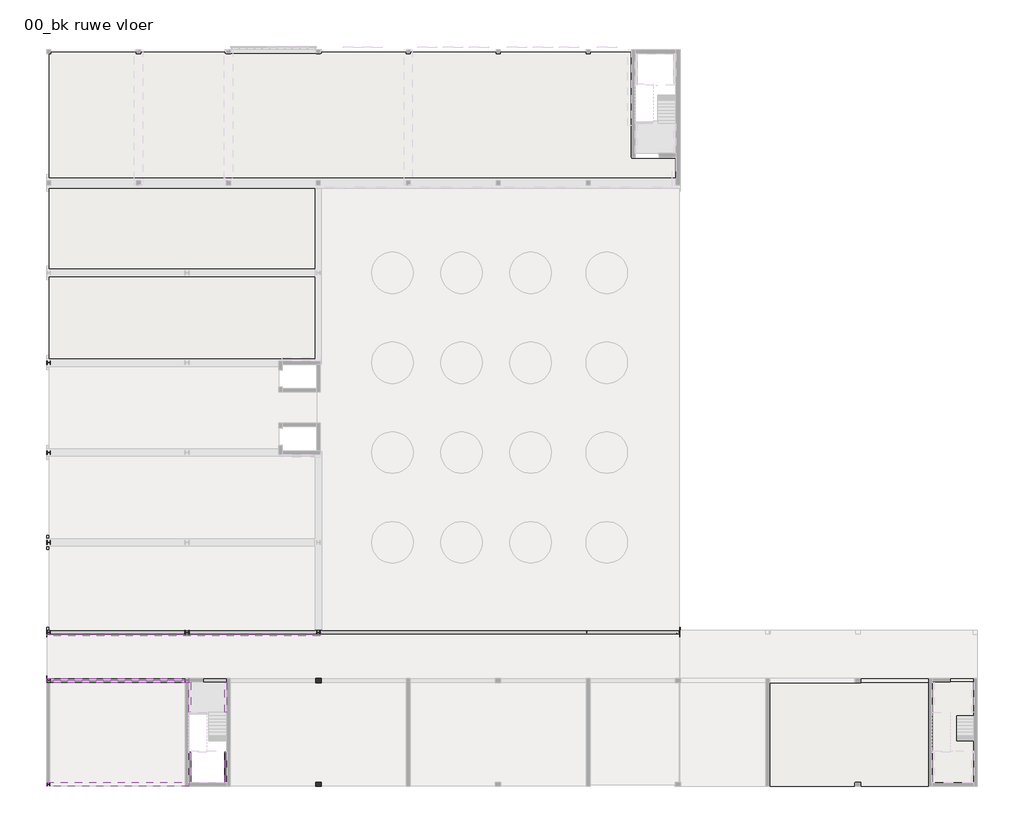
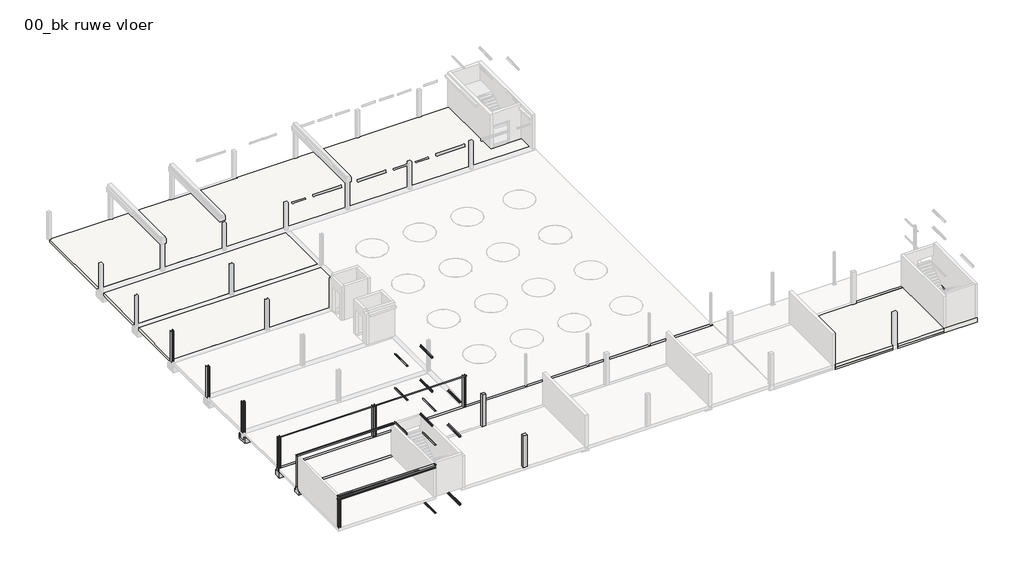
# One storey, part 4 of 6: 24 beams, 10 columns, 8 slabs.
"""IFC4 building model written with IfcOpenShell, lengths in millimetres."""

import ifcopenshell
import ifcopenshell.guid

model = None  # the IFC model being written
_history = None  # IfcOwnerHistory: only IFC2X3 demands one
_inside = {}  # id of a spatial element -> (the spatial element, [elements in it])
_under = {}  # id of a project, library or spatial element -> (it, [spatial elements below it])
_declared = {}  # id of a project -> (the project, [libraries it declares])
_typed = {}  # id of a type object -> (the type object, [elements of that type])
_made_of = {}  # id of a material, layer set ... -> (it, [elements and type objects made of it])


def new_model(schema):
    """Start an empty IFC model of exactly this schema.

    Asked for "IFC4X3", IfcOpenShell would pick the latest addendum, in which some entities
    have other attributes; the version numbers below select the first issue.
    IFC2X3 requires an IfcOwnerHistory on every rooted entity: one is made here for all.
    """
    global model, _history
    if schema == "IFC4X3":
        model = ifcopenshell.file(schema_version=(4, 3, 0, 0))
    else:
        model = ifcopenshell.file(schema=schema)
    _inside.clear()
    _under.clear()
    _declared.clear()
    _typed.clear()
    _made_of.clear()
    _history = None
    if model.schema == "IFC2X3":
        org = make("IfcOrganization", Name="unknown")
        user = make(
            "IfcPersonAndOrganization",
            ThePerson=make("IfcPerson", FamilyName="unknown"),
            TheOrganization=org,
        )
        app = make(
            "IfcApplication",
            ApplicationDeveloper=org,
            Version="unknown",
            ApplicationFullName="unknown",
            ApplicationIdentifier="unknown",
        )
        _history = make(
            "IfcOwnerHistory",
            OwningUser=user,
            OwningApplication=app,
            ChangeAction="ADDED",
            CreationDate=0,
        )
    return model


def make(cls, **values):
    """One entity of the class cls with the attributes given. An attribute that is None is left unset."""
    return model.create_entity(
        cls, **{name: value for name, value in values.items() if value is not None}
    )


def rooted(cls, **values):
    """An entity with a GlobalId (a new one), such as an element, a storey or a relation."""
    return make(cls, GlobalId=ifcopenshell.guid.new(), OwnerHistory=_history, **values)


def si_unit(unit_type, name, prefix=None):
    """IfcSIUnit, for example si_unit("LENGTHUNIT", "METRE", prefix="MILLI")."""
    return make("IfcSIUnit", UnitType=unit_type, Prefix=prefix, Name=name)


def assignment(units):
    """IfcUnitAssignment: the units of a project."""
    return None if units is None else make("IfcUnitAssignment", Units=units)


def point(xyz):
    """IfcCartesianPoint."""
    return None if xyz is None else make("IfcCartesianPoint", Coordinates=xyz)


def direction(xyz):
    """IfcDirection."""
    return None if xyz is None else make("IfcDirection", DirectionRatios=xyz)


def frame(location, z_axis=None, x_axis=None):
    """IfcAxis2Placement3D, a coordinate frame: its origin and axes. An axis left out is left unset."""
    return make(
        "IfcAxis2Placement3D",
        Location=point(location),
        Axis=direction(z_axis),
        RefDirection=direction(x_axis),
    )


def frame_2d(location, x_axis=None):
    """IfcAxis2Placement2D, a coordinate frame in the plane: its origin and x axis."""
    return make(
        "IfcAxis2Placement2D", Location=point(location), RefDirection=direction(x_axis)
    )


def origin():
    """The frame at (0, 0, 0) with its axes left unset."""
    return frame((0.0, 0.0, 0.0))


def place(relative_to, where):
    """IfcLocalPlacement: puts the frame where relative to a parent placement (None: the world)."""
    return make(
        "IfcLocalPlacement", PlacementRelTo=relative_to, RelativePlacement=where
    )


def context(
    kind, dimensions, precision=None, world=None, true_north=None, identifier=None
):
    """IfcGeometricRepresentationContext, for example the 3D "Model" context."""
    return make(
        "IfcGeometricRepresentationContext",
        ContextIdentifier=identifier,
        ContextType=kind,
        CoordinateSpaceDimension=dimensions,
        Precision=precision,
        WorldCoordinateSystem=world,
        TrueNorth=true_north,
    )


def project(units=None, contexts=None):
    """IfcProject with its units and contexts."""
    return rooted(
        "IfcProject",
        Name="project",
        RepresentationContexts=contexts,
        UnitsInContext=assignment(units),
    )


def spatial(cls, under=None, at=None, **own):
    """A site, building, storey or space (cls), placed at a placement, below another one or the project."""
    s = rooted(cls, ObjectPlacement=at, **own)
    if under is not None:
        _under.setdefault(under.id(), (under, []))[1].append(s)
    return s


def polyline(points):
    """IfcPolyline through the points."""
    return make("IfcPolyline", Points=[point(p) for p in points])


def circle_curve(where, radius):
    """IfcCircle in the frame where."""
    return make("IfcCircle", Position=where, Radius=radius)


def trimmed(basis, trim1, trim2, sense, master):
    """IfcTrimmedCurve: the piece of a basis curve between two trims."""
    return make(
        "IfcTrimmedCurve",
        BasisCurve=basis,
        Trim1=trim1,
        Trim2=trim2,
        SenseAgreement=sense,
        MasterRepresentation=master,
    )


def segment(curve, same_sense, transition):
    """IfcCompositeCurveSegment."""
    return make(
        "IfcCompositeCurveSegment",
        Transition=transition,
        SameSense=same_sense,
        ParentCurve=curve,
    )


def composite_curve(segments, self_intersect=None):
    """IfcCompositeCurve: segments joined end to end."""
    return make("IfcCompositeCurve", Segments=segments, SelfIntersect=self_intersect)


def outline(outer, holes=None, kind="AREA"):
    """IfcArbitraryClosedProfileDef: a profile drawn as a closed curve; with holes, ...WithVoids."""
    if holes is None:
        return make("IfcArbitraryClosedProfileDef", ProfileType=kind, OuterCurve=outer)
    return make(
        "IfcArbitraryProfileDefWithVoids",
        ProfileType=kind,
        OuterCurve=outer,
        InnerCurves=holes,
    )


def extrude(swept, where, along, depth):
    """IfcExtrudedAreaSolid: the profile swept, set in the frame where, extruded along a direction by depth."""
    return make(
        "IfcExtrudedAreaSolid",
        SweptArea=swept,
        Position=where,
        ExtrudedDirection=direction(along),
        Depth=depth,
    )


def faces_of(points, faces, orient=None, outer=None):
    """IfcFace entities. A face is a list of loops; a loop is a list of indices into points, from 0.

    orient and outer hold one flag for each loop. By default every Orientation is true, the
    first loop of a face is its IfcFaceOuterBound and the others are IfcFaceBound.
    """
    made = []
    for i, loops in enumerate(faces):
        bounds = []
        for j, loop in enumerate(loops):
            is_outer = j == 0 if outer is None else outer[i][j]
            bounds.append(
                make(
                    "IfcFaceOuterBound" if is_outer else "IfcFaceBound",
                    Bound=make("IfcPolyLoop", Polygon=[points[k] for k in loop]),
                    Orientation=True if orient is None else orient[i][j],
                )
            )
        made.append(make("IfcFace", Bounds=bounds))
    return made


def faceted_brep(points, faces, orient=None, outer=None, voids=None):
    """IfcFacetedBrep: a solid bounded by flat faces; with voids (closed shells), ...WithVoids."""
    shared = [point(p) for p in points]
    hull = make("IfcClosedShell", CfsFaces=faces_of(shared, faces, orient, outer))
    if voids is None:
        return make("IfcFacetedBrep", Outer=hull)
    return make(
        "IfcFacetedBrepWithVoids",
        Outer=hull,
        Voids=[
            make(cls, CfsFaces=faces_of(shared, fs, o, b)) for cls, fs, o, b in voids
        ],
    )


def shape(context_of_items, identifier, shape_type, items):
    """IfcShapeRepresentation: the items that make up one representation, for example the "Body"."""
    return make(
        "IfcShapeRepresentation",
        ContextOfItems=context_of_items,
        RepresentationIdentifier=identifier,
        RepresentationType=shape_type,
        Items=items,
    )


def source(mapping_origin, context_of_items, identifier, shape_type, items):
    """IfcRepresentationMap: a shape defined once, which mapped items show again and again."""
    return make(
        "IfcRepresentationMap",
        MappingOrigin=mapping_origin,
        MappedRepresentation=shape(context_of_items, identifier, shape_type, items),
    )


def transform(
    local_origin,
    x_axis=None,
    y_axis=None,
    z_axis=None,
    scale=None,
    scale2=None,
    scale3=None,
    uniform=True,
):
    """IfcCartesianTransformationOperator3D, or its non-uniform kind. x_axis, y_axis, z_axis: its Axis1, 2, 3."""
    if uniform:
        return make(
            "IfcCartesianTransformationOperator3D",
            Axis1=direction(x_axis),
            Axis2=direction(y_axis),
            LocalOrigin=point(local_origin),
            Scale=scale,
            Axis3=direction(z_axis),
        )
    return make(
        "IfcCartesianTransformationOperator3DnonUniform",
        Axis1=direction(x_axis),
        Axis2=direction(y_axis),
        LocalOrigin=point(local_origin),
        Scale=scale,
        Axis3=direction(z_axis),
        Scale2=scale2,
        Scale3=scale3,
    )


def mapped(mapping_source, mapping_target):
    """IfcMappedItem: shows the shape of a source again, moved by a transform."""
    return make(
        "IfcMappedItem", MappingSource=mapping_source, MappingTarget=mapping_target
    )


def made_of(thing, what):
    """Note that an element or type object is made of a material, layer set ...; save() writes the relation."""
    if what is not None:
        _made_of.setdefault(what.id(), (what, []))[1].append(thing)
    return thing


def element(
    cls,
    number,
    at=None,
    inside=None,
    cuts=None,
    type_object=None,
    material=None,
    context=None,
    identifier="Body",
    shape_type=None,
    held_by="IfcProductDefinitionShape",
    body=None,
    shapes=None,
    **own,
):
    """One element of the class cls, such as IfcWall. Its Tag is "e" and its number.

    at: its placement. inside: the storey or other place that contains it. cuts: it is an
    opening in that element (IfcRelVoidsElement). A single representation is given by context,
    identifier, shape_type and body (its items); several are given by shapes. held_by: the class
    of the entity that holds the representations. save() writes the other relations.
    """
    e = rooted(cls, Tag="e%d" % number, ObjectPlacement=at, **own)
    if body is not None:
        shapes = [shape(context, identifier, shape_type, body)]
    if shapes is not None:
        e.Representation = make(held_by, Representations=shapes)
    if inside is not None:
        _inside.setdefault(inside.id(), (inside, []))[1].append(e)
    if cuts is not None:
        rooted(
            "IfcRelVoidsElement", RelatingBuildingElement=cuts, RelatedOpeningElement=e
        )
    if type_object is not None:
        _typed.setdefault(type_object.id(), (type_object, []))[1].append(e)
    return made_of(e, material)


def aggregate(whole, parts):
    """IfcRelAggregates: a whole, such as a stair, and the parts it consists of."""
    return rooted("IfcRelAggregates", RelatingObject=whole, RelatedObjects=parts)


def save(model, path):
    """Write the relations noted so far, then the file.

    IfcRelAggregates (storeys below a building ...), IfcRelContainedInSpatialStructure (elements
    in a storey), IfcRelDefinesByType, IfcRelAssociatesMaterial and IfcRelDeclares: one each for
    every whole, place, type object, material and project.
    """
    for whole, parts in _under.values():
        aggregate(whole, parts)
    for where, things in _inside.values():
        rooted(
            "IfcRelContainedInSpatialStructure",
            RelatedElements=things,
            RelatingStructure=where,
        )
    for kind, things in _typed.values():
        rooted("IfcRelDefinesByType", RelatedObjects=things, RelatingType=kind)
    for what, things in _made_of.values():
        rooted("IfcRelAssociatesMaterial", RelatedObjects=things, RelatingMaterial=what)
    for by, libraries in _declared.values():
        rooted("IfcRelDeclares", RelatingContext=by, RelatedDefinitions=libraries)
    model.write(path)


def beam_86464b0d(model_context):
    return source(origin(), model_context, "Body", "SweptSolid", [
        extrude(outline(composite_curve([segment(polyline([(-42.5, -42.5), (-42.5, 107.5), (-35.5, 107.5)]), True, "CONTINUOUS"), segment(trimmed(circle_curve(frame_2d((-35.5, 99.5)), 8.0), [point((-35.5, 107.5))], [point((-27.5, 99.5))], False, "CARTESIAN"), True, "CONTINUOUS"), segment(polyline([(-27.5, 99.5), (-27.5, -11.5)]), True, "CONTINUOUS"), segment(trimmed(circle_curve(frame_2d((-11.5, -11.5)), 16.0), [point((-27.5, -11.5))], [point((-11.5, -27.5))], True, "CARTESIAN"), True, "CONTINUOUS"), segment(polyline([(-11.5, -27.5), (99.5, -27.5)]), True, "CONTINUOUS"), segment(trimmed(circle_curve(frame_2d((99.5, -35.5)), 8.0), [point((99.5, -27.5))], [point((107.5, -35.5))], False, "CARTESIAN"), True, "CONTINUOUS"), segment(polyline([(107.5, -35.5), (107.5, -42.5), (-42.5, -42.5)]), True, "CONTINUOUS")], self_intersect=False)), frame((-1095.0, 0.0, 0.0), z_axis=(1.0, 0.0, 0.0), x_axis=(0.0, 1.0, 0.0)), (0.0, 0.0, 1.0), 2190.0),
    ])


def beam_a9a0024c(model_context):
    return source(origin(), model_context, "Body", "SweptSolid", [
        extrude(outline(composite_curve([segment(polyline([(42.5, -42.5), (-107.5, -42.5), (-107.5, -35.5)]), True, "CONTINUOUS"), segment(trimmed(circle_curve(frame_2d((-99.5, -35.5)), 8.0), [point((-107.5, -35.5))], [point((-99.5, -27.5))], False, "CARTESIAN"), True, "CONTINUOUS"), segment(polyline([(-99.5, -27.5), (11.5, -27.5)]), True, "CONTINUOUS"), segment(trimmed(circle_curve(frame_2d((11.5, -11.5)), 16.0), [point((11.5, -27.5))], [point((27.5, -11.5))], True, "CARTESIAN"), True, "CONTINUOUS"), segment(polyline([(27.5, -11.5), (27.5, 99.5)]), True, "CONTINUOUS"), segment(trimmed(circle_curve(frame_2d((35.5, 99.5)), 8.0), [point((27.5, 99.5))], [point((35.5, 107.5))], False, "CARTESIAN"), True, "CONTINUOUS"), segment(polyline([(35.5, 107.5), (42.5, 107.5), (42.5, -42.5)]), True, "CONTINUOUS")], self_intersect=False)), frame((-1095.0, 0.0, 0.0), z_axis=(1.0, 0.0, 0.0), x_axis=(0.0, 1.0, 0.0)), (0.0, 0.0, 1.0), 2190.0),
    ])


model = new_model("IFC4")

# Units and contexts
model_context = context("Model", 3, world=origin())
ifc_project = project(units=[si_unit("LENGTHUNIT", "METRE", prefix="MILLI")], contexts=[model_context])

# Site, building, storey
site = spatial("IfcSite", under=ifc_project)
building = spatial("IfcBuilding", under=site)
storey = spatial("IfcBuildingStorey", under=building, Name="00_bk ruwe vloer", Elevation=-70.0)

# Beams
placement = place(None, origin())
element("IfcBeam", 1, ObjectType="NLRS_28_SF_LIB_balk dubbele sponning beton prefab-CWV-MMBC-SRP_gen_rsf : balk beton prefab_gen__bxh 700x900 met inkassing bxh 200x320", at=placement, inside=storey, context=model_context, shape_type="Brep", body=[
    faceted_brep([(52150.0, 11150.0, -70.0), (52150.0, 10850.0, -70.0), (52150.0, 10850.0, -390.0), (52150.0, 10650.0, -390.0), (52150.0, 10650.0, -970.0), (52150.0, 11350.0, -970.0), (52150.0, 11350.0, -390.0), (52150.0, 11150.0, -390.0), (6350.0, 11150.0, -70.0), (6350.0, 11150.0, -390.0), (6350.0, 11350.0, -390.0), (6350.0, 11350.0, -970.0), (6350.0, 10650.0, -970.0), (6350.0, 10650.0, -390.0), (6350.0, 10850.0, -390.0), (6350.0, 10850.0, -70.0), (52090.0, 11150.0, -70.0), (26300.0, 11150.0, -70.0), (25750.0, 11150.0, -70.0), (6550.0, 11150.0, -70.0), (6410.0, 10850.0, -70.0), (52090.0, 10850.0, -70.0), (6410.0, 10850.0, -390.0), (52090.0, 10850.0, -390.0), (6410.0, 10650.0, -390.0), (6625.0, 10650.0, -390.0), (6650.0, 10650.0, -390.0), (51850.0, 10650.0, -390.0), (51875.0, 10650.0, -390.0), (52090.0, 10650.0, -390.0), (6650.0, 10650.0, -970.0), (51850.0, 10650.0, -970.0), (6650.0, 11350.0, -970.0), (25500.0, 11350.0, -970.0), (26500.0, 11350.0, -970.0), (51850.0, 11350.0, -970.0), (6550.0, 11350.0, -390.0), (6650.0, 11350.0, -390.0), (25500.0, 11350.0, -390.0), (25750.0, 11350.0, -390.0), (26300.0, 11350.0, -390.0), (26425.0, 11350.0, -390.0), (26500.0, 11350.0, -390.0), (51850.0, 11350.0, -390.0), (51875.0, 11350.0, -390.0), (52090.0, 11350.0, -390.0), (6550.0, 11150.0, -390.0), (25750.0, 11150.0, -390.0), (26300.0, 11150.0, -390.0), (52090.0, 11150.0, -390.0)], [[[0, 1, 2, 3, 4, 5, 6, 7]], [[8, 9, 10, 11, 12, 13, 14, 15]], [[1, 0, 16, 17, 18, 19, 8, 15, 20, 21]], [[2, 1, 21, 20, 15, 14, 22, 23]], [[3, 2, 23, 22, 14, 13, 24, 25, 26, 27, 28, 29]], [[4, 3, 29, 28, 27, 26, 25, 24, 13, 12, 30, 31]], [[5, 4, 31, 30, 12, 11, 32, 33, 34, 35]], [[6, 5, 35, 34, 33, 32, 11, 10, 36, 37, 38, 39, 40, 41, 42, 43, 44, 45]], [[7, 6, 45, 44, 43, 42, 41, 40, 39, 38, 37, 36, 10, 9, 46, 47, 48, 49]], [[0, 7, 49, 48, 47, 46, 9, 8, 19, 18, 17, 16]]]),
])
element("IfcBeam", 2, ObjectType="NLRS_28_SF_LIB_balkbodem beton prefab-CWV-MMBC-SRP_gen_rsf : balkbodem beton prefab_gen__bxhxdk 1000x580x200", at=placement, inside=storey, context=model_context, shape_type="Brep", body=[
    faceted_brep([(25550.0, 17000.0, -390.0), (25550.0, 17000.0, -970.0), (25550.0, 18000.0, -970.0), (25550.0, 18000.0, -390.0), (25550.0, 17800.0, -390.0), (25550.0, 17800.0, -770.0), (25550.0, 17200.0, -770.0), (25550.0, 17200.0, -390.0), (6350.0, 17000.0, -390.0), (6350.0, 17200.0, -390.0), (6350.0, 17200.0, -770.0), (6350.0, 17800.0, -770.0), (6350.0, 17800.0, -390.0), (6350.0, 18000.0, -390.0), (6350.0, 18000.0, -970.0), (6350.0, 17000.0, -970.0), (25500.0, 17000.0, -390.0), (6650.0, 17000.0, -390.0), (6550.0, 17000.0, -390.0), (6650.0, 17000.0, -970.0), (25500.0, 17000.0, -970.0), (6650.0, 18000.0, -970.0), (25500.0, 18000.0, -970.0), (6550.0, 18000.0, -390.0), (6650.0, 18000.0, -390.0), (25500.0, 18000.0, -390.0), (6550.0, 17800.0, -390.0), (25500.0, 17800.0, -390.0), (25500.0, 17800.0, -770.0), (25500.0, 17200.0, -770.0), (6550.0, 17200.0, -390.0), (25500.0, 17200.0, -390.0)], [[[0, 1, 2, 3, 4, 5, 6, 7]], [[8, 9, 10, 11, 12, 13, 14, 15]], [[1, 0, 16, 17, 18, 8, 15, 19, 20]], [[2, 1, 20, 19, 15, 14, 21, 22]], [[3, 2, 22, 21, 14, 13, 23, 24, 25]], [[4, 3, 25, 24, 23, 13, 12, 26, 27]], [[5, 4, 27, 26, 12, 11, 28]], [[6, 5, 28, 11, 10, 29]], [[7, 6, 29, 10, 9, 30, 31]], [[0, 7, 31, 30, 9, 8, 18, 17, 16]]]),
])
element("IfcBeam", 3, ObjectType="NLRS_28_SF_LIB_balk dubbele sponning beton prefab-CWV-MMBC-SRP_gen_rsf : balk beton prefab_gen__bxh 700x700 met inkassing bxh 200x320", at=placement, inside=storey, context=model_context, shape_type="Brep", body=[
    faceted_brep([(6350.0, 7650.0, -70.0), (6350.0, 7650.0, -390.0), (6350.0, 7850.0, -390.0), (6350.0, 7850.0, -770.0), (6350.0, 7150.0, -770.0), (6350.0, 7150.0, -390.0), (6350.0, 7350.0, -390.0), (6350.0, 7350.0, -70.0), (6410.0, 7350.0, -70.0), (16625.0, 7350.0, -70.0), (16625.0, 7400.0, -70.0), (16625.0, 7650.0, -70.0), (16375.0, 7650.0, -70.0), (6410.0, 7650.0, -70.0), (6410.0, 7350.0, -390.0), (16375.0, 7350.0, -390.0), (16625.0, 7350.0, -390.0), (6410.0, 7150.0, -390.0), (6625.0, 7150.0, -390.0), (6650.0, 7150.0, -390.0), (16375.0, 7150.0, -390.0), (6650.0, 7150.0, -770.0), (16375.0, 7150.0, -770.0), (6650.0, 7850.0, -770.0), (16625.0, 7850.0, -770.0), (16625.0, 7650.0, -770.0), (16375.0, 7650.0, -770.0), (6410.0, 7850.0, -390.0), (6625.0, 7850.0, -390.0), (6650.0, 7850.0, -390.0), (16625.0, 7850.0, -390.0), (6410.0, 7650.0, -390.0), (16375.0, 7650.0, -390.0), (16625.0, 7650.0, -390.0), (16625.0, 7825.0, -390.0), (16375.0, 7650.0, -390.0)], [[[0, 1, 2, 3, 4, 5, 6, 7]], [[0, 7, 8, 9, 10, 11, 12, 13]], [[7, 6, 14, 15, 16, 9, 8]], [[6, 5, 17, 18, 19, 20, 15, 14]], [[5, 4, 21, 22, 20, 19, 18, 17]], [[4, 3, 23, 24, 25, 26, 22, 21]], [[3, 2, 27, 28, 29, 30, 24, 23]], [[2, 1, 31, 32, 33, 34, 30, 29, 28, 27]], [[1, 0, 13, 12, 11, 33, 32, 31]], [[11, 10, 9, 16, 33]], [[35, 15, 20, 22, 26]], [[35, 33, 16, 15]], [[33, 35, 26, 25]], [[24, 30, 34, 33, 25]]]),
])
element("IfcBeam", 4, ObjectType="NLRS_28_SF_LIB_balk dubbele sponning beton prefab-CWV-MMBC-SRP_gen_rsf : balk beton prefab_gen__bxh 700x700 met inkassing bxh 200x320", at=placement, inside=storey, context=model_context, shape_type="Brep", body=[
    faceted_brep([(16625.0, 7650.0, -70.0), (16625.0, 7650.0, -390.0), (16625.0, 7825.0, -390.0), (16625.0, 7850.0, -390.0), (16625.0, 7850.0, -770.0), (16625.0, 7650.0, -770.0), (16625.0, 7400.0, -770.0), (16625.0, 7400.0, -70.0), (17675.0, 7400.0, -70.0), (19375.0, 7400.0, -70.0), (19375.0, 7650.0, -70.0), (17675.0, 7650.0, -70.0), (19375.0, 7850.0, -770.0), (19375.0, 7650.0, -770.0), (19375.0, 7400.0, -770.0), (19375.0, 7850.0, -390.0), (19375.0, 7650.0, -390.0), (19375.0, 7825.0, -390.0)], [[[0, 1, 2, 3, 4, 5, 6, 7]], [[0, 7, 8, 9, 10, 11]], [[6, 5, 4, 12, 13, 14]], [[4, 3, 15, 12]], [[15, 3, 2, 1, 16, 17]], [[1, 0, 11, 10, 16]], [[7, 6, 14, 9, 8]], [[10, 9, 14, 13, 12, 15, 17, 16]]]),
])
element("IfcBeam", 5, ObjectType="NLRS_28_SF_LIB_stalen ligger HEB-AV-CWV-MMBS-SRP_gen_rsf : stalen ligger_gen__HEB 360", at=placement, inside=storey, context=model_context, shape_type="SweptSolid", body=[
    extrude(outline(composite_curve([segment(polyline([(150.0, 3447.5), (33.25, 3447.5)]), True, "CONTINUOUS"), segment(trimmed(circle_curve(frame_2d((33.25, 3420.5)), 27.0), [point((33.25, 3447.5))], [point((6.25, 3420.5))], True, "CARTESIAN"), True, "CONTINUOUS"), segment(polyline([(6.25, 3420.5), (6.25, 3159.5)]), True, "CONTINUOUS"), segment(trimmed(circle_curve(frame_2d((33.25, 3159.5)), 27.0), [point((6.25, 3159.5))], [point((33.25, 3132.5))], True, "CARTESIAN"), True, "CONTINUOUS"), segment(polyline([(33.25, 3132.5), (150.0, 3132.5), (150.0, 3110.0), (-150.0, 3110.0), (-150.0, 3132.5), (-33.25, 3132.5)]), True, "CONTINUOUS"), segment(trimmed(circle_curve(frame_2d((-33.25, 3159.5)), 27.0), [point((-33.25, 3132.5))], [point((-6.25, 3159.5))], True, "CARTESIAN"), True, "CONTINUOUS"), segment(polyline([(-6.25, 3159.5), (-6.25, 3420.5)]), True, "CONTINUOUS"), segment(trimmed(circle_curve(frame_2d((-33.25, 3420.5)), 27.0), [point((-6.25, 3420.5))], [point((-33.25, 3447.5))], True, "CARTESIAN"), True, "CONTINUOUS"), segment(polyline([(-33.25, 3447.5), (-150.0, 3447.5), (-150.0, 3470.0), (150.0, 3470.0), (150.0, 3447.5)]), True, "CONTINUOUS")], self_intersect=False)), frame((6350.0, 0.0, 0.0), z_axis=(1.0, 0.0, 0.0), x_axis=(0.0, 1.0, 0.0)), (0.0, 0.0, 1.0), 10275.0),
])
element("IfcBeam", 6, ObjectType="NLRS_28_SF_LIB_stalen ligger stripstaal-AV-MMBS-SRP_gen_rsf : stalen ligger stripstaal RECT_gen__140x15", at=placement, inside=storey, context=model_context, shape_type="SweptSolid", body=[
    extrude(outline(polyline([(16625.0, 7493.0), (16625.0, 7353.0), (6350.0, 7353.0), (6350.0, 7493.0), (16625.0, 7493.0)])), frame((0.0, 0.0, 3455.0), z_axis=(0.0, 0.0, 1.0), x_axis=(1.0, 0.0, 0.0)), (0.0, 0.0, 1.0), 15.0),
    extrude(outline(polyline([(16625.0, 7493.0), (16625.0, 7353.0), (6350.0, 7353.0), (6350.0, 7493.0), (16625.0, 7493.0)])), frame((0.0, 0.0, 3455.0), z_axis=(0.0, 0.0, 1.0), x_axis=(1.0, 0.0, 0.0)), (0.0, 0.0, 1.0), 15.0),
])
element("IfcBeam", 7, ObjectType="NLRS_28_SF_LIB_stalen ligger stripstaal-AV-MMBS-SRP_gen_rsf : stalen ligger stripstaal RECT_gen__140x15", at=placement, inside=storey, context=model_context, shape_type="SweptSolid", body=[
    extrude(outline(polyline([(16625.0, 7507.0), (6350.0, 7507.0), (6350.0, 7647.0), (16625.0, 7647.0), (16625.0, 7507.0)])), frame((0.0, 0.0, 3455.0), z_axis=(0.0, 0.0, 1.0), x_axis=(1.0, 0.0, 0.0)), (0.0, 0.0, 1.0), 15.0),
    extrude(outline(polyline([(16625.0, 7507.0), (6350.0, 7507.0), (6350.0, 7647.0), (16625.0, 7647.0), (16625.0, 7507.0)])), frame((0.0, 0.0, 3455.0), z_axis=(0.0, 0.0, 1.0), x_axis=(1.0, 0.0, 0.0)), (0.0, 0.0, 1.0), 15.0),
])
element("IfcBeam", 8, ObjectType="NLRS_28_SF_LIB_stalen ligger stripstaal-AV-MMBS-SRP_gen_rsf : stalen ligger stripstaal RECT_gen__120x15", at=placement, inside=storey, context=model_context, shape_type="SweptSolid", body=[
    extrude(outline(polyline([(26125.0, 10856.5), (26125.0, 10736.5), (6350.0, 10736.5), (6350.0, 10856.5), (26125.0, 10856.5)])), frame((0.0, 0.0, 3455.0), z_axis=(0.0, 0.0, 1.0), x_axis=(1.0, 0.0, 0.0)), (0.0, 0.0, 1.0), 15.0),
    extrude(outline(polyline([(26125.0, 10856.5), (26125.0, 10736.5), (6350.0, 10736.5), (6350.0, 10856.5), (26125.0, 10856.5)])), frame((0.0, 0.0, 3455.0), z_axis=(0.0, 0.0, 1.0), x_axis=(1.0, 0.0, 0.0)), (0.0, 0.0, 1.0), 15.0),
])
beam_shape = beam_86464b0d(model_context)
element("IfcBeam", 9, ObjectType="NLRS_28_SF_LIB_stalen ligger hoekprofiel gelijkzijdig-AV-MMBS-SRP_gen_rsf : stalen ligger gelijkzijdig hoekprofiel LEQU_gen__150x150x15", at=placement, inside=storey, context=model_context, shape_type="MappedRepresentation", body=[
    mapped(beam_shape, transform((19332.5, 1205.0, 1722.5), x_axis=(0.0, 1.0, 0.0), y_axis=(-1.0, 0.0, 0.0), z_axis=(0.0, 0.0, 1.0))),
])
element("IfcBeam", 10, ObjectType="NLRS_28_SF_LIB_stalen ligger hoekprofiel gelijkzijdig-AV-MMBS-SRP_gen_rsf : stalen ligger gelijkzijdig hoekprofiel LEQU_gen__150x150x15", at=placement, inside=storey, context=model_context, shape_type="MappedRepresentation", body=[
    mapped(beam_shape, transform((19332.5, 1205.0, -2077.5), x_axis=(0.0, 1.0, 0.0), y_axis=(-1.0, 0.0, 0.0), z_axis=(0.0, 0.0, 1.0))),
])
element("IfcBeam", 11, ObjectType="NLRS_28_SF_LIB_stalen ligger hoekprofiel gelijkzijdig-AV-MMBS-SRP_gen_rsf : stalen ligger gelijkzijdig hoekprofiel LEQU_gen__150x150x15", at=placement, inside=storey, context=model_context, shape_type="MappedRepresentation", body=[
    mapped(beam_shape, transform((19332.5, 1205.0, 5522.5), x_axis=(0.0, 1.0, 0.0), y_axis=(-1.0, 0.0, 0.0), z_axis=(0.0, 0.0, 1.0))),
])
element("IfcBeam", 12, ObjectType="NLRS_28_SF_LIB_stalen ligger hoekprofiel gelijkzijdig-AV-MMBS-SRP_gen_rsf : stalen ligger gelijkzijdig hoekprofiel LEQU_gen__150x150x15", at=placement, inside=storey, context=model_context, shape_type="MappedRepresentation", body=[
    mapped(beam_shape, transform((19332.5, 1205.0, 9322.5), x_axis=(0.0, 1.0, 0.0), y_axis=(-1.0, 0.0, 0.0), z_axis=(0.0, 0.0, 1.0))),
])
element("IfcBeam", 13, ObjectType="NLRS_28_SF_LIB_stalen ligger hoekprofiel gelijkzijdig-AV-MMBS-SRP_gen_rsf : stalen ligger gelijkzijdig hoekprofiel LEQU_gen__150x150x15", at=placement, inside=storey, context=model_context, shape_type="MappedRepresentation", body=[
    mapped(beam_shape, transform((19332.5, 6295.0, -177.5), x_axis=(0.0, 1.0, 0.0), y_axis=(-1.0, 0.0, 0.0), z_axis=(0.0, 0.0, 1.0))),
])
element("IfcBeam", 14, ObjectType="NLRS_28_SF_LIB_stalen ligger hoekprofiel gelijkzijdig-AV-MMBS-SRP_gen_rsf : stalen ligger gelijkzijdig hoekprofiel LEQU_gen__150x150x15", at=placement, inside=storey, context=model_context, shape_type="MappedRepresentation", body=[
    mapped(beam_shape, transform((19332.5, 6295.0, 3622.5), x_axis=(0.0, 1.0, 0.0), y_axis=(-1.0, 0.0, 0.0), z_axis=(0.0, 0.0, 1.0))),
])
element("IfcBeam", 15, ObjectType="NLRS_28_SF_LIB_stalen ligger hoekprofiel gelijkzijdig-AV-MMBS-SRP_gen_rsf : stalen ligger gelijkzijdig hoekprofiel LEQU_gen__150x150x15", at=placement, inside=storey, context=model_context, shape_type="MappedRepresentation", body=[
    mapped(beam_shape, transform((19332.5, 6295.0, 7422.5), x_axis=(0.0, 1.0, 0.0), y_axis=(-1.0, 0.0, 0.0), z_axis=(0.0, 0.0, 1.0))),
])
element("IfcBeam", 16, ObjectType="NLRS_28_SF_LIB_stalen ligger hoekprofiel gelijkzijdig-AV-MMBS-SRP_gen_rsf : stalen ligger gelijkzijdig hoekprofiel LEQU_gen__150x150x15", at=placement, inside=storey, context=model_context, shape_type="MappedRepresentation", body=[
    mapped(beam_shape, transform((19332.5, 6295.0, 11222.5), x_axis=(0.0, 1.0, 0.0), y_axis=(-1.0, 0.0, 0.0), z_axis=(0.0, 0.0, 1.0))),
])
beam_2_shape = beam_a9a0024c(model_context)
element("IfcBeam", 17, ObjectType="NLRS_28_SF_LIB_stalen ligger hoekprofiel gelijkzijdig-AV-MMBS-SRP_gen_rsf : stalen ligger gelijkzijdig hoekprofiel LEQU_gen__150x150x15", at=placement, inside=storey, context=model_context, shape_type="MappedRepresentation", body=[
    mapped(beam_2_shape, transform((16667.5, 1205.0, 1722.5), x_axis=(0.0, 1.0, 0.0), y_axis=(-1.0, 0.0, 0.0), z_axis=(0.0, 0.0, 1.0))),
])
element("IfcBeam", 18, ObjectType="NLRS_28_SF_LIB_stalen ligger hoekprofiel gelijkzijdig-AV-MMBS-SRP_gen_rsf : stalen ligger gelijkzijdig hoekprofiel LEQU_gen__150x150x15", at=placement, inside=storey, context=model_context, shape_type="MappedRepresentation", body=[
    mapped(beam_2_shape, transform((16667.5, 1205.0, -2077.5), x_axis=(0.0, 1.0, 0.0), y_axis=(-1.0, 0.0, 0.0), z_axis=(0.0, 0.0, 1.0))),
])
element("IfcBeam", 19, ObjectType="NLRS_28_SF_LIB_stalen ligger hoekprofiel gelijkzijdig-AV-MMBS-SRP_gen_rsf : stalen ligger gelijkzijdig hoekprofiel LEQU_gen__150x150x15", at=placement, inside=storey, context=model_context, shape_type="MappedRepresentation", body=[
    mapped(beam_2_shape, transform((16667.5, 1205.0, 5522.5), x_axis=(0.0, 1.0, 0.0), y_axis=(-1.0, 0.0, 0.0), z_axis=(0.0, 0.0, 1.0))),
])
element("IfcBeam", 20, ObjectType="NLRS_28_SF_LIB_stalen ligger hoekprofiel gelijkzijdig-AV-MMBS-SRP_gen_rsf : stalen ligger gelijkzijdig hoekprofiel LEQU_gen__150x150x15", at=placement, inside=storey, context=model_context, shape_type="MappedRepresentation", body=[
    mapped(beam_2_shape, transform((16667.5, 1205.0, 9322.5), x_axis=(0.0, 1.0, 0.0), y_axis=(-1.0, 0.0, 0.0), z_axis=(0.0, 0.0, 1.0))),
])
element("IfcBeam", 21, ObjectType="NLRS_28_SF_LIB_stalen ligger hoekprofiel gelijkzijdig-AV-MMBS-SRP_gen_rsf : stalen ligger gelijkzijdig hoekprofiel LEQU_gen__150x150x15", at=placement, inside=storey, context=model_context, shape_type="MappedRepresentation", body=[
    mapped(beam_2_shape, transform((16667.5, 6295.0, -177.5), x_axis=(0.0, 1.0, 0.0), y_axis=(-1.0, 0.0, 0.0), z_axis=(0.0, 0.0, 1.0))),
])
element("IfcBeam", 22, ObjectType="NLRS_28_SF_LIB_stalen ligger hoekprofiel gelijkzijdig-AV-MMBS-SRP_gen_rsf : stalen ligger gelijkzijdig hoekprofiel LEQU_gen__150x150x15", at=placement, inside=storey, context=model_context, shape_type="MappedRepresentation", body=[
    mapped(beam_2_shape, transform((16667.5, 6295.0, 3622.5), x_axis=(0.0, 1.0, 0.0), y_axis=(-1.0, 0.0, 0.0), z_axis=(0.0, 0.0, 1.0))),
])
element("IfcBeam", 23, ObjectType="NLRS_28_SF_LIB_stalen ligger hoekprofiel gelijkzijdig-AV-MMBS-SRP_gen_rsf : stalen ligger gelijkzijdig hoekprofiel LEQU_gen__150x150x15", at=placement, inside=storey, context=model_context, shape_type="MappedRepresentation", body=[
    mapped(beam_2_shape, transform((16667.5, 6295.0, 7422.5), x_axis=(0.0, 1.0, 0.0), y_axis=(-1.0, 0.0, 0.0), z_axis=(0.0, 0.0, 1.0))),
])
element("IfcBeam", 24, ObjectType="NLRS_28_SF_LIB_stalen ligger hoekprofiel gelijkzijdig-AV-MMBS-SRP_gen_rsf : stalen ligger gelijkzijdig hoekprofiel LEQU_gen__150x150x15", at=placement, inside=storey, context=model_context, shape_type="MappedRepresentation", body=[
    mapped(beam_2_shape, transform((16667.5, 6295.0, 11222.5), x_axis=(0.0, 1.0, 0.0), y_axis=(-1.0, 0.0, 0.0), z_axis=(0.0, 0.0, 1.0))),
])

# Columns
element("IfcColumn", 25, ObjectType="NLRS_28_SCO_TLB_stalen kolom HEA-BCPG-MMBS-SRP_gen_rsf : stalen kolom_gen__HEA 260", at=placement, inside=storey, context=model_context, shape_type="SweptSolid", body=[
    extrude(outline(composite_curve([segment(polyline([(6375.0, 11130.0), (6387.5, 11130.0), (6387.5, 11027.75)]), True, "CONTINUOUS"), segment(trimmed(circle_curve(frame_2d((6411.5, 11027.75)), 24.0), [point((6387.5, 11027.75))], [point((6411.5, 11003.75))], True, "CARTESIAN"), True, "CONTINUOUS"), segment(polyline([(6411.5, 11003.75), (6588.5, 11003.75)]), True, "CONTINUOUS"), segment(trimmed(circle_curve(frame_2d((6588.5, 11027.75)), 24.0), [point((6588.5, 11003.75))], [point((6612.5, 11027.75))], True, "CARTESIAN"), True, "CONTINUOUS"), segment(polyline([(6612.5, 11027.75), (6612.5, 11130.0), (6625.0, 11130.0), (6625.0, 10870.0), (6612.5, 10870.0), (6612.5, 10972.25)]), True, "CONTINUOUS"), segment(trimmed(circle_curve(frame_2d((6588.5, 10972.25)), 24.0), [point((6612.5, 10972.25))], [point((6588.5, 10996.25))], True, "CARTESIAN"), True, "CONTINUOUS"), segment(polyline([(6588.5, 10996.25), (6411.5, 10996.25)]), True, "CONTINUOUS"), segment(trimmed(circle_curve(frame_2d((6411.5, 10972.25)), 24.0), [point((6411.5, 10996.25))], [point((6387.5, 10972.25))], True, "CARTESIAN"), True, "CONTINUOUS"), segment(polyline([(6387.5, 10972.25), (6387.5, 10870.0), (6375.0, 10870.0), (6375.0, 11130.0)]), True, "CONTINUOUS")], self_intersect=False)), frame((0.0, 0.0, -40.0), z_axis=(0.0, 0.0, 1.0), x_axis=(1.0, 0.0, 0.0)), (0.0, 0.0, 1.0), 3420.0),
])
element("IfcColumn", 26, ObjectType="NLRS_28_SCO_TLB_stalen kolom HEA-BCPG-MMBS-SRP_gen_rsf : stalen kolom_gen__HEA 260", at=placement, inside=storey, context=model_context, shape_type="SweptSolid", body=[
    extrude(outline(composite_curve([segment(polyline([(6375.0, 17630.0), (6387.5, 17630.0), (6387.5, 17527.75)]), True, "CONTINUOUS"), segment(trimmed(circle_curve(frame_2d((6411.5, 17527.75)), 24.0), [point((6387.5, 17527.75))], [point((6411.5, 17503.75))], True, "CARTESIAN"), True, "CONTINUOUS"), segment(polyline([(6411.5, 17503.75), (6588.5, 17503.75)]), True, "CONTINUOUS"), segment(trimmed(circle_curve(frame_2d((6588.5, 17527.75)), 24.0), [point((6588.5, 17503.75))], [point((6612.5, 17527.75))], True, "CARTESIAN"), True, "CONTINUOUS"), segment(polyline([(6612.5, 17527.75), (6612.5, 17630.0), (6625.0, 17630.0), (6625.0, 17370.0), (6612.5, 17370.0), (6612.5, 17472.25)]), True, "CONTINUOUS"), segment(trimmed(circle_curve(frame_2d((6588.5, 17472.25)), 24.0), [point((6612.5, 17472.25))], [point((6588.5, 17496.25))], True, "CARTESIAN"), True, "CONTINUOUS"), segment(polyline([(6588.5, 17496.25), (6411.5, 17496.25)]), True, "CONTINUOUS"), segment(trimmed(circle_curve(frame_2d((6411.5, 17472.25)), 24.0), [point((6411.5, 17496.25))], [point((6387.5, 17472.25))], True, "CARTESIAN"), True, "CONTINUOUS"), segment(polyline([(6387.5, 17472.25), (6387.5, 17370.0), (6375.0, 17370.0), (6375.0, 17630.0)]), True, "CONTINUOUS")], self_intersect=False)), frame((0.0, 0.0, -40.0), z_axis=(0.0, 0.0, 1.0), x_axis=(1.0, 0.0, 0.0)), (0.0, 0.0, 1.0), 3420.0),
])
element("IfcColumn", 27, ObjectType="NLRS_28_SCO_TLB_stalen kolom HEA-BCPG-MMBS-SRP_gen_rsf : stalen kolom_gen__HEA 260", at=placement, inside=storey, context=model_context, shape_type="SweptSolid", body=[
    extrude(outline(composite_curve([segment(polyline([(6375.0, 24130.0), (6387.5, 24130.0), (6387.5, 24027.75)]), True, "CONTINUOUS"), segment(trimmed(circle_curve(frame_2d((6411.5, 24027.75)), 24.0), [point((6387.5, 24027.75))], [point((6411.5, 24003.75))], True, "CARTESIAN"), True, "CONTINUOUS"), segment(polyline([(6411.5, 24003.75), (6588.5, 24003.75)]), True, "CONTINUOUS"), segment(trimmed(circle_curve(frame_2d((6588.5, 24027.75)), 24.0), [point((6588.5, 24003.75))], [point((6612.5, 24027.75))], True, "CARTESIAN"), True, "CONTINUOUS"), segment(polyline([(6612.5, 24027.75), (6612.5, 24130.0), (6625.0, 24130.0), (6625.0, 23870.0), (6612.5, 23870.0), (6612.5, 23972.25)]), True, "CONTINUOUS"), segment(trimmed(circle_curve(frame_2d((6588.5, 23972.25)), 24.0), [point((6612.5, 23972.25))], [point((6588.5, 23996.25))], True, "CARTESIAN"), True, "CONTINUOUS"), segment(polyline([(6588.5, 23996.25), (6411.5, 23996.25)]), True, "CONTINUOUS"), segment(trimmed(circle_curve(frame_2d((6411.5, 23972.25)), 24.0), [point((6411.5, 23996.25))], [point((6387.5, 23972.25))], True, "CARTESIAN"), True, "CONTINUOUS"), segment(polyline([(6387.5, 23972.25), (6387.5, 23870.0), (6375.0, 23870.0), (6375.0, 24130.0)]), True, "CONTINUOUS")], self_intersect=False)), frame((0.0, 0.0, -40.0), z_axis=(0.0, 0.0, 1.0), x_axis=(1.0, 0.0, 0.0)), (0.0, 0.0, 1.0), 3420.0),
])
element("IfcColumn", 28, ObjectType="NLRS_28_SCO_TLB_stalen kolom HEA-BCPG-MMBS-SRP_gen_rsf : stalen kolom_gen__HEA 260", at=placement, inside=storey, context=model_context, shape_type="SweptSolid", body=[
    extrude(outline(composite_curve([segment(polyline([(6375.0, 30630.0), (6387.5, 30630.0), (6387.5, 30527.75)]), True, "CONTINUOUS"), segment(trimmed(circle_curve(frame_2d((6411.5, 30527.75)), 24.0), [point((6387.5, 30527.75))], [point((6411.5, 30503.75))], True, "CARTESIAN"), True, "CONTINUOUS"), segment(polyline([(6411.5, 30503.75), (6588.5, 30503.75)]), True, "CONTINUOUS"), segment(trimmed(circle_curve(frame_2d((6588.5, 30527.75)), 24.0), [point((6588.5, 30503.75))], [point((6612.5, 30527.75))], True, "CARTESIAN"), True, "CONTINUOUS"), segment(polyline([(6612.5, 30527.75), (6612.5, 30630.0), (6625.0, 30630.0), (6625.0, 30370.0), (6612.5, 30370.0), (6612.5, 30472.25)]), True, "CONTINUOUS"), segment(trimmed(circle_curve(frame_2d((6588.5, 30472.25)), 24.0), [point((6612.5, 30472.25))], [point((6588.5, 30496.25))], True, "CARTESIAN"), True, "CONTINUOUS"), segment(polyline([(6588.5, 30496.25), (6411.5, 30496.25)]), True, "CONTINUOUS"), segment(trimmed(circle_curve(frame_2d((6411.5, 30472.25)), 24.0), [point((6411.5, 30496.25))], [point((6387.5, 30472.25))], True, "CARTESIAN"), True, "CONTINUOUS"), segment(polyline([(6387.5, 30472.25), (6387.5, 30370.0), (6375.0, 30370.0), (6375.0, 30630.0)]), True, "CONTINUOUS")], self_intersect=False)), frame((0.0, 0.0, -40.0), z_axis=(0.0, 0.0, 1.0), x_axis=(1.0, 0.0, 0.0)), (0.0, 0.0, 1.0), 3420.0),
])
element("IfcColumn", 29, ObjectType="NLRS_28_SCO_TLB_stalen kolom HEB-BCPG-MMBS-SRP_gen_rsf : stalen kolom_gen__HEB 300", at=placement, inside=storey, context=model_context, shape_type="SweptSolid", body=[
    extrude(outline(composite_curve([segment(polyline([(16350.0, 11150.0), (16369.0, 11150.0), (16369.0, 11032.5)]), True, "CONTINUOUS"), segment(trimmed(circle_curve(frame_2d((16396.0, 11032.5)), 27.0), [point((16369.0, 11032.5))], [point((16396.0, 11005.5))], True, "CARTESIAN"), True, "CONTINUOUS"), segment(polyline([(16396.0, 11005.5), (16604.0, 11005.5)]), True, "CONTINUOUS"), segment(trimmed(circle_curve(frame_2d((16604.0, 11032.5)), 27.0), [point((16604.0, 11005.5))], [point((16631.0, 11032.5))], True, "CARTESIAN"), True, "CONTINUOUS"), segment(polyline([(16631.0, 11032.5), (16631.0, 11150.0), (16650.0, 11150.0), (16650.0, 10850.0), (16631.0, 10850.0), (16631.0, 10967.5)]), True, "CONTINUOUS"), segment(trimmed(circle_curve(frame_2d((16604.0, 10967.5)), 27.0), [point((16631.0, 10967.5))], [point((16604.0, 10994.5))], True, "CARTESIAN"), True, "CONTINUOUS"), segment(polyline([(16604.0, 10994.5), (16396.0, 10994.5)]), True, "CONTINUOUS"), segment(trimmed(circle_curve(frame_2d((16396.0, 10967.5)), 27.0), [point((16396.0, 10994.5))], [point((16369.0, 10967.5))], True, "CARTESIAN"), True, "CONTINUOUS"), segment(polyline([(16369.0, 10967.5), (16369.0, 10850.0), (16350.0, 10850.0), (16350.0, 11150.0)]), True, "CONTINUOUS")], self_intersect=False)), frame((0.0, 0.0, -40.0), z_axis=(0.0, 0.0, 1.0), x_axis=(1.0, 0.0, 0.0)), (0.0, 0.0, 1.0), 3420.0),
])
element("IfcColumn", 30, ObjectType="NLRS_28_SCO_TLB_stalen kolom HEA-BCPG-MMBS-SRP_gen_rsf : stalen kolom_gen__HEA 260", at=placement, inside=storey, context=model_context, shape_type="SweptSolid", body=[
    extrude(outline(composite_curve([segment(polyline([(25875.0, 11130.0), (25887.5, 11130.0), (25887.5, 11027.75)]), True, "CONTINUOUS"), segment(trimmed(circle_curve(frame_2d((25911.5, 11027.75)), 24.0), [point((25887.5, 11027.75))], [point((25911.5, 11003.75))], True, "CARTESIAN"), True, "CONTINUOUS"), segment(polyline([(25911.5, 11003.75), (26088.5, 11003.75)]), True, "CONTINUOUS"), segment(trimmed(circle_curve(frame_2d((26088.5, 11027.75)), 24.0), [point((26088.5, 11003.75))], [point((26112.5, 11027.75))], True, "CARTESIAN"), True, "CONTINUOUS"), segment(polyline([(26112.5, 11027.75), (26112.5, 11130.0), (26125.0, 11130.0), (26125.0, 10870.0), (26112.5, 10870.0), (26112.5, 10972.25)]), True, "CONTINUOUS"), segment(trimmed(circle_curve(frame_2d((26088.5, 10972.25)), 24.0), [point((26112.5, 10972.25))], [point((26088.5, 10996.25))], True, "CARTESIAN"), True, "CONTINUOUS"), segment(polyline([(26088.5, 10996.25), (25911.5, 10996.25)]), True, "CONTINUOUS"), segment(trimmed(circle_curve(frame_2d((25911.5, 10972.25)), 24.0), [point((25911.5, 10996.25))], [point((25887.5, 10972.25))], True, "CARTESIAN"), True, "CONTINUOUS"), segment(polyline([(25887.5, 10972.25), (25887.5, 10870.0), (25875.0, 10870.0), (25875.0, 11130.0)]), True, "CONTINUOUS")], self_intersect=False)), frame((0.0, 0.0, -40.0), z_axis=(0.0, 0.0, 1.0), x_axis=(1.0, 0.0, 0.0)), (0.0, 0.0, 1.0), 3420.0),
])
element("IfcColumn", 31, ObjectType="NLRS_28_SCO_TLB_vierkante kolom beton ihwg-BCPG-MMBC-SRP_gen_rsf : vierkante kolom beton ihwg_gen__bxh 400x300", at=placement, inside=storey, context=model_context, shape_type="SweptSolid", body=[
    extrude(outline(polyline([(26200.0, 7650.0), (26200.0, 7350.0), (25800.0, 7350.0), (25800.0, 7650.0), (26200.0, 7650.0)])), frame((0.0, 0.0, -70.0), z_axis=(0.0, 0.0, 1.0), x_axis=(1.0, 0.0, 0.0)), (0.0, 0.0, 1.0), 3540.0),
])
element("IfcColumn", 32, ObjectType="NLRS_28_SCO_TLB_vierkante kolom beton ihwg-BCPG-MMBC-SRP_gen_rsf : vierkante kolom beton ihwg_gen__bxh 400x300", at=placement, inside=storey, context=model_context, shape_type="SweptSolid", body=[
    extrude(outline(polyline([(26200.0, 150.0), (26200.0, -150.0), (25800.0, -150.0), (25800.0, 150.0), (26200.0, 150.0)])), frame((0.0, 0.0, -70.0), z_axis=(0.0, 0.0, 1.0), x_axis=(1.0, 0.0, 0.0)), (0.0, 0.0, 1.0), 3540.0),
])
element("IfcColumn", 33, ObjectType="NLRS_28_SCO_TLB_stalen kolom HEA-BCPG-MMBS-SRP_gen_rsf : stalen kolom_gen__HEA 240", at=placement, inside=storey, context=model_context, shape_type="SweptSolid", body=[
    extrude(outline(composite_curve([segment(polyline([(6385.0, 7620.0), (6397.0, 7620.0), (6397.0, 7524.75)]), True, "CONTINUOUS"), segment(trimmed(circle_curve(frame_2d((6418.0, 7524.75)), 21.0), [point((6397.0, 7524.75))], [point((6418.0, 7503.75))], True, "CARTESIAN"), True, "CONTINUOUS"), segment(polyline([(6418.0, 7503.75), (6582.0, 7503.75)]), True, "CONTINUOUS"), segment(trimmed(circle_curve(frame_2d((6582.0, 7524.75)), 21.0), [point((6582.0, 7503.75))], [point((6603.0, 7524.75))], True, "CARTESIAN"), True, "CONTINUOUS"), segment(polyline([(6603.0, 7524.75), (6603.0, 7620.0), (6615.0, 7620.0), (6615.0, 7380.0), (6603.0, 7380.0), (6603.0, 7475.25)]), True, "CONTINUOUS"), segment(trimmed(circle_curve(frame_2d((6582.0, 7475.25)), 21.0), [point((6603.0, 7475.25))], [point((6582.0, 7496.25))], True, "CARTESIAN"), True, "CONTINUOUS"), segment(polyline([(6582.0, 7496.25), (6418.0, 7496.25)]), True, "CONTINUOUS"), segment(trimmed(circle_curve(frame_2d((6418.0, 7475.25)), 21.0), [point((6418.0, 7496.25))], [point((6397.0, 7475.25))], True, "CARTESIAN"), True, "CONTINUOUS"), segment(polyline([(6397.0, 7475.25), (6397.0, 7380.0), (6385.0, 7380.0), (6385.0, 7620.0)]), True, "CONTINUOUS")], self_intersect=False)), frame((0.0, 0.0, -40.0), z_axis=(0.0, 0.0, 1.0), x_axis=(1.0, 0.0, 0.0)), (0.0, 0.0, 1.0), 3390.0),
])
element("IfcColumn", 34, ObjectType="NLRS_28_SCO_TLB_stalen kolom HEA-BCPG-MMBS-SRP_gen_rsf : stalen kolom_gen__HEA 200", at=placement, inside=storey, context=model_context, shape_type="SweptSolid", body=[
    extrude(outline(composite_curve([segment(polyline([(6405.0, 100.0), (6415.0, 100.0), (6415.0, 21.25)]), True, "CONTINUOUS"), segment(trimmed(circle_curve(frame_2d((6433.0, 21.25)), 18.0), [point((6415.0, 21.25))], [point((6433.0, 3.25))], True, "CARTESIAN"), True, "CONTINUOUS"), segment(polyline([(6433.0, 3.25), (6567.0, 3.25)]), True, "CONTINUOUS"), segment(trimmed(circle_curve(frame_2d((6567.0, 21.25)), 18.0), [point((6567.0, 3.25))], [point((6585.0, 21.25))], True, "CARTESIAN"), True, "CONTINUOUS"), segment(polyline([(6585.0, 21.25), (6585.0, 100.0), (6595.0, 100.0), (6595.0, -100.0), (6585.0, -100.0), (6585.0, -21.25)]), True, "CONTINUOUS"), segment(trimmed(circle_curve(frame_2d((6567.0, -21.25)), 18.0), [point((6585.0, -21.25))], [point((6567.0, -3.25))], True, "CARTESIAN"), True, "CONTINUOUS"), segment(polyline([(6567.0, -3.25), (6433.0, -3.25)]), True, "CONTINUOUS"), segment(trimmed(circle_curve(frame_2d((6433.0, -21.25)), 18.0), [point((6433.0, -3.25))], [point((6415.0, -21.25))], True, "CARTESIAN"), True, "CONTINUOUS"), segment(polyline([(6415.0, -21.25), (6415.0, -100.0), (6405.0, -100.0), (6405.0, 100.0)]), True, "CONTINUOUS")], self_intersect=False)), frame((0.0, 0.0, -40.0), z_axis=(0.0, 0.0, 1.0), x_axis=(1.0, 0.0, 0.0)), (0.0, 0.0, 1.0), 3150.0),
])

# Slabs
element("IfcSlab", 35, ObjectType="NLRS_23_FL_isolatieplaatvloer 320_gen_rsf", at=placement, inside=storey, context=model_context, shape_type="SweptSolid", body=[
    extrude(outline(polyline([(64750.0, 7350.0), (64750.0, 7300.0), (65250.0, 7300.0), (65250.0, 7350.0), (70125.0, 7350.0), (70125.0, -150.0), (65250.0, -150.0), (65250.0, 150.0), (64750.0, 150.0), (64750.0, -150.0), (58650.0, -150.0), (58650.0, 7350.0), (64750.0, 7350.0)])), frame((0.0, 0.0, -390.0), z_axis=(0.0, 0.0, 1.0), x_axis=(1.0, 0.0, 0.0)), (0.0, 0.0, 1.0), 320.0),
])
element("IfcSlab", 36, ObjectType="NLRS_23_FL_isolatieplaatvloer 320_gen_rsf", at=placement, inside=storey, context=model_context, shape_type="SweptSolid", body=[
    extrude(outline(polyline([(73400.0, 7400.0), (73400.0, 100.0), (70375.0, 100.0), (70375.0, 7400.0), (73400.0, 7400.0)])), frame((0.0, 0.0, -390.0), z_axis=(0.0, 0.0, 1.0), x_axis=(1.0, 0.0, 0.0)), (0.0, 0.0, 1.0), 320.0),
])
element("IfcSlab", 37, ObjectType="NLRS_23_FL_isolatieplaatvloer 320_gen_rsf", at=placement, inside=storey, context=model_context, shape_type="Brep", body=[
    faceted_brep([(25750.0, 36700.0, -390.0), (25750.0, 30800.0, -390.0), (25550.0, 30800.0, -390.0), (6550.0, 30800.0, -390.0), (6550.0, 31000.0, -390.0), (6550.0, 36500.0, -390.0), (6550.0, 36700.0, -390.0), (25550.0, 36700.0, -390.0), (25750.0, 36700.0, -70.0), (6550.0, 36700.0, -70.0), (6550.0, 30800.0, -70.0), (25750.0, 30800.0, -70.0)], [[[0, 1, 2, 3, 4, 5, 6, 7]], [[8, 9, 10, 11]], [[1, 0, 8, 11]], [[3, 2, 1, 11, 10]], [[6, 5, 4, 3, 10, 9]], [[0, 7, 6, 9, 8]]]),
])
element("IfcSlab", 38, ObjectType="NLRS_23_FL_isolatieplaatvloer 320_gen_rsf", at=placement, inside=storey, context=model_context, shape_type="Brep", body=[
    faceted_brep([(25750.0, 43100.0, -390.0), (25750.0, 42900.0, -390.0), (25750.0, 37300.0, -390.0), (25550.0, 37300.0, -390.0), (6550.0, 37300.0, -390.0), (6550.0, 37500.0, -390.0), (6550.0, 42900.0, -390.0), (6550.0, 43100.0, -390.0), (25750.0, 43100.0, -70.0), (6550.0, 43100.0, -70.0), (6550.0, 37300.0, -70.0), (25750.0, 37300.0, -70.0)], [[[0, 1, 2, 3, 4, 5, 6, 7]], [[8, 9, 10, 11]], [[2, 1, 0, 8, 11]], [[4, 3, 2, 11, 10]], [[7, 6, 5, 4, 10, 9]], [[0, 7, 9, 8]]]),
])
element("IfcSlab", 39, ObjectType="NLRS_23_FL_isolatieplaatvloer 320_gen_rsf", at=placement, inside=storey, context=model_context, shape_type="Brep", body=[
    faceted_brep([(19250.0, 52950.0, -390.0), (19250.0, 52850.0, -390.0), (26250.0, 52850.0, -390.0), (26250.0, 52950.0, -390.0), (48605.0, 52950.0, -390.0), (48605.0, 52850.0, -390.0), (48605.0, 45270.0, -390.0), (51850.0, 45270.0, -390.0), (51950.0, 45270.0, -390.0), (51950.0, 44100.0, -390.0), (51950.0, 43900.0, -390.0), (6550.0, 43900.0, -390.0), (6550.0, 44100.0, -390.0), (6550.0, 52950.0, -390.0), (6650.0, 52950.0, -390.0), (19250.0, 52950.0, -70.0), (6650.0, 52950.0, -70.0), (6550.0, 52950.0, -70.0), (6550.0, 43900.0, -70.0), (51950.0, 43900.0, -70.0), (51950.0, 45270.0, -70.0), (51850.0, 45270.0, -70.0), (48605.0, 45270.0, -70.0), (48605.0, 52850.0, -70.0), (48605.0, 52950.0, -70.0), (26250.0, 52950.0, -70.0), (26250.0, 52850.0, -70.0), (19250.0, 52850.0, -70.0)], [[[0, 1, 2, 3, 4, 5, 6, 7, 8, 9, 10, 11, 12, 13, 14]], [[15, 16, 17, 18, 19, 20, 21, 22, 23, 24, 25, 26, 27]], [[10, 9, 8, 20, 19]], [[11, 10, 19, 18]], [[13, 12, 11, 18, 17]], [[0, 14, 13, 17, 16, 15]], [[6, 5, 4, 24, 23, 22]], [[8, 7, 6, 22, 21, 20]], [[1, 0, 15, 27]], [[2, 1, 27, 26]], [[3, 2, 26, 25]], [[4, 3, 25, 24]]]),
])
element("IfcSlab", 40, ObjectType="NLRS_23_FL_beton ihwg vloeraanstort 520_gen_rsf", at=placement, inside=storey, context=model_context, shape_type="Brep", body=[
    faceted_brep([(73650.0, 7650.0, -590.0), (73650.0, -150.0, -590.0), (70125.0, -150.0, -590.0), (70125.0, 7350.0, -590.0), (65250.0, 7350.0, -590.0), (65250.0, 7650.0, -590.0), (73400.0, 7400.0, -590.0), (70375.0, 7400.0, -590.0), (70375.0, 100.0, -590.0), (73400.0, 100.0, -590.0), (73650.0, 7650.0, -70.0), (73400.0, 7650.0, -70.0), (71700.0, 7650.0, -70.0), (70375.0, 7650.0, -70.0), (70125.0, 7650.0, -70.0), (65250.0, 7650.0, -70.0), (65250.0, 7350.0, -70.0), (70125.0, 7350.0, -70.0), (70125.0, -150.0, -70.0), (70375.0, -150.0, -70.0), (73400.0, -150.0, -70.0), (73650.0, -150.0, -70.0), (73400.0, 7400.0, -70.0), (73400.0, 100.0, -70.0), (70375.0, 100.0, -70.0), (70375.0, 7400.0, -70.0), (71700.0, 7400.0, -70.0)], [[[0, 1, 2, 3, 4, 5], [6, 7, 8, 9]], [[10, 11, 12, 13, 14, 15, 16, 17, 18, 19, 20, 21], [22, 23, 24, 25, 26]], [[1, 0, 10, 21]], [[2, 1, 21, 20, 19, 18]], [[3, 2, 18, 17]], [[4, 3, 17, 16]], [[5, 4, 16, 15]], [[0, 5, 15, 14, 13, 12, 11, 10]], [[7, 6, 22, 26, 25]], [[8, 7, 25, 24]], [[9, 8, 24, 23]], [[6, 9, 23, 22]]]),
])
element("IfcSlab", 41, ObjectType="NLRS_23_FL_isolatie isolatieplaatvloer 200_gen_rsf", at=placement, inside=storey, context=model_context, shape_type="SweptSolid", body=[
    extrude(outline(polyline([(64750.0, 7350.0), (64750.0, 7300.0), (65250.0, 7300.0), (65250.0, 7350.0), (70125.0, 7350.0), (70125.0, -150.0), (65250.0, -150.0), (65250.0, 150.0), (64750.0, 150.0), (64750.0, -150.0), (58650.0, -150.0), (58650.0, 7350.0), (64750.0, 7350.0)])), frame((0.0, 0.0, -590.0), z_axis=(0.0, 0.0, 1.0), x_axis=(1.0, 0.0, 0.0)), (0.0, 0.0, 1.0), 200.0),
])
element("IfcSlab", 42, ObjectType="NLRS_23_FL_isolatie isolatieplaatvloer 200_gen_rsf", at=placement, inside=storey, context=model_context, shape_type="SweptSolid", body=[
    extrude(outline(polyline([(73400.0, 7400.0), (73400.0, 100.0), (70375.0, 100.0), (70375.0, 7400.0), (73400.0, 7400.0)])), frame((0.0, 0.0, -590.0), z_axis=(0.0, 0.0, 1.0), x_axis=(1.0, 0.0, 0.0)), (0.0, 0.0, 1.0), 200.0),
])

save(model, "model.ifc")

# Revit data of these elements
# Type "NLRS_28_SF_LIB_balk dubbele sponning beton prefab-CWV-MMBC-SRP_gen_rsf : balk beton prefab_gen__bxh 700x900 met inkassing bxh 200x320"
#   Type IfcGUID = "3VXE8Tiz5F69n85q0kAzGV"
#   IfcExportAs = "IfcBeamType"
#   Type Comments = "700x900"
#   Description = "balk beton ihwg 700x900 dubbele inkassing 200x320"
#   Assembly Code = "28.11"
#   RSF_C_hoogte_inkassing_rechts = 320 mm
#   RSF_C_hoogte_inkassing_links = 320 mm
#   RSF_C_breedte_inkassing_rechts = 200 mm
#   RSF_C_breedte_inkassing_links = 200 mm
#   NLRS_C_lengte [instance default] = 3000 mm
#   NLRS_C_hoogte = 900 mm
#   NLRS_C_breedte = 700 mm
#   Length [instance default] = 3000 mm
#   Structural Material = NLRS_f2_beton prefab_gen_rsf
#   Model = ""
# Type "NLRS_28_SF_LIB_balkbodem beton prefab-CWV-MMBC-SRP_gen_rsf : balkbodem beton prefab_gen__bxhxdk 1000x580x200"
#   Type IfcGUID = "0X0KViByb4JPBOa4XaNhJR"
#   IfcExportAs = "IfcBeamType"
#   Type Comments = "1000x580"
#   Description = "balkbodem beton prefab 1000x580"
#   Assembly Code = "28.11"
#   NLRS_C_lengte [instance default] = 3000 mm
#   NLRS_C_hoogte = 580 mm
#   NLRS_C_dikte = 200 mm
#   NLRS_C_breedte = 1000 mm
#   Length [instance default] = 3000 mm
#   Structural Material = NLRS_f2_beton prefab_gen_rsf
#   Model = ""
# Type "NLRS_28_SF_LIB_balk dubbele sponning beton prefab-CWV-MMBC-SRP_gen_rsf : balk beton prefab_gen__bxh 700x700 met inkassing bxh 200x320"
#   Type IfcGUID = "3Qemsd6Xj1WRJeMYmB12mi"
#   IfcExportAs = "IfcBeamType"
#   Type Comments = "700x700"
#   Description = "balk beton ihwg 700x700 dubbele inkassing 200x320"
#   Assembly Code = "28.11"
#   RSF_C_hoogte_inkassing_rechts = 320 mm
#   RSF_C_hoogte_inkassing_links = 320 mm
#   RSF_C_breedte_inkassing_rechts = 200 mm
#   RSF_C_breedte_inkassing_links = 200 mm
#   NLRS_C_lengte [instance default] = 3000 mm
#   NLRS_C_hoogte = 700 mm
#   NLRS_C_breedte = 700 mm
#   Length [instance default] = 3000 mm
#   Structural Material = NLRS_f2_beton prefab_gen_rsf
#   Model = ""
# Type "NLRS_28_SF_LIB_stalen ligger HEB-AV-CWV-MMBS-SRP_gen_rsf : stalen ligger_gen__HEB 360"
#   Type IfcGUID = "0zo1UjqZ91lRsfCKsOOa5E"
#   IfcExportAs = "IfcBeamType"
#   Type Comments = "HEB360"
#   Model = " "
#   Manufacturer = " "
#   Fire Rating = " "
#   Description = "stalen ligger HEB360"
#   Assembly Code = "28.11"
#   ra = 27 mm
#   vz = 180 mm
#   vy = 150 mm
#   vpz = 180 mm
#   vpy = 150 mm
#   NLRS_C_lengte [instance default] = 1500 mm
#   Length [instance default] = 1500 mm
#   bf = 300 mm
#   d = 360 mm
#   tf = 22.5 mm
#   tw = 12.5 mm
#   Structural Material = NLRS_h2_staal_gen_rsf
#   Keynote = ""
# Type "NLRS_28_SF_LIB_stalen ligger stripstaal-AV-MMBS-SRP_gen_rsf : stalen ligger stripstaal RECT_gen__140x15"
#   Type IfcGUID = "00ECIG4lbEgBwDs3wwpa4k"
#   IfcExportAs = "IfcBeamType"
#   Type Comments = "strip140x15"
#   Model = " "
#   Manufacturer = " "
#   Fire Rating = " "
#   Description = "stalen ligger strip140x15"
#   Assembly Code = "28.11"
#   vz = 7.5 mm
#   vy = 70 mm
#   vpz = 7.5 mm
#   vpy = 70 mm
#   NLRS_C_lengte [instance default] = 1500 mm
#   Length [instance default] = 1500 mm
#   bf = 140 mm
#   d = 15 mm
#   Structural Material = NLRS_h2_staal_gen_rsf
#   Keynote = ""
# Type "NLRS_28_SF_LIB_stalen ligger stripstaal-AV-MMBS-SRP_gen_rsf : stalen ligger stripstaal RECT_gen__120x15"
#   Type IfcGUID = "00ECIG4lbEgBwDs3wwpa4w"
#   IfcExportAs = "IfcBeamType"
#   Type Comments = "strip120x15"
#   Model = " "
#   Manufacturer = " "
#   Fire Rating = " "
#   Description = "stalen ligger strip 120x15"
#   Assembly Code = "28.11"
#   vz = 7.5 mm
#   vy = 60 mm
#   vpz = 7.5 mm
#   vpy = 60 mm
